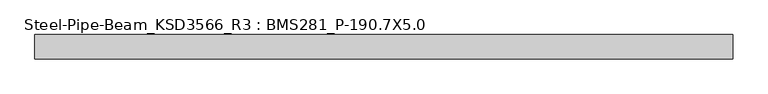
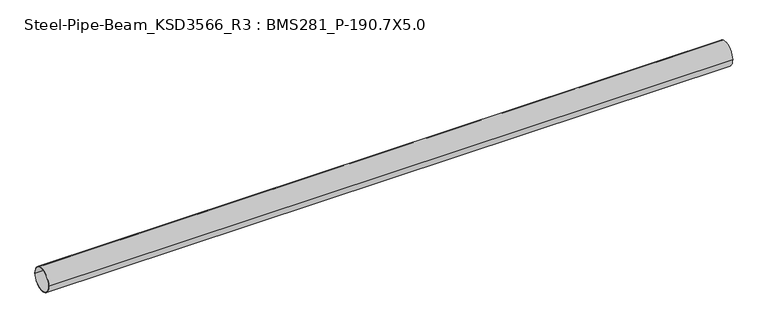
"""IFC4 building model written with IfcOpenShell, lengths in millimetres: member geometry, Steel-Pipe-Beam_KSD3566_R3 : BMS281_P-190.7X5.0."""

from ifc_helpers import new_model, si_unit, point, frame, origin, origin_2d, place, context, project, spatial, circle_curve, trimmed, segment, composite_curve, outline, extrude, source, transform, mapped, element, save


def steel_pipe_beam_ksd3566_r3_bms281_p_190_7x5_0_8f12f416(model_context):
    return source(origin(), model_context, "Body", "SweptSolid", [
        extrude(outline(composite_curve([segment(trimmed(circle_curve(origin_2d(), 95.35), [point((-95.35, 0.0))], [point((95.35, 0.0))], False, "CARTESIAN"), True, "CONTINUOUS"), segment(trimmed(circle_curve(origin_2d(), 95.35), [point((95.35, 0.0))], [point((-95.35, 0.0))], False, "CARTESIAN"), True, "CONTINUOUS")], self_intersect=False), holes=[composite_curve([segment(trimmed(circle_curve(origin_2d(), 90.35), [point((90.35, 0.0))], [point((-90.35, 0.0))], True, "CARTESIAN"), True, "CONTINUOUS"), segment(trimmed(circle_curve(origin_2d(), 90.35), [point((-90.35, 0.0))], [point((90.35, 0.0))], True, "CARTESIAN"), True, "CONTINUOUS")], self_intersect=False)]), frame((-2743.0186842, 0.0, 0.0), z_axis=(1.0, 0.0, 0.0), x_axis=(0.0, 1.0, 0.0)), (0.0, 0.0, 1.0), 5479.06158),
    ])


if __name__ == "__main__":
    model = new_model("IFC4")
    model_context = context("Model", 3, world=origin())
    ifc_project = project(units=[si_unit("LENGTHUNIT", "METRE", prefix="MILLI")], contexts=[model_context])
    site = spatial("IfcSite", under=ifc_project)
    building = spatial("IfcBuilding", under=site)
    placement = place(None, origin())
    steel_pipe_beam_ksd3566_r3_bms281_p_190_7x5_0_shape = steel_pipe_beam_ksd3566_r3_bms281_p_190_7x5_0_8f12f416(model_context)
    element("IfcMember", 1, ObjectType="Steel-Pipe-Beam_KSD3566_R3 : BMS281_P-190.7X5.0", at=placement, inside=building, context=model_context, shape_type="MappedRepresentation", body=[
        mapped(steel_pipe_beam_ksd3566_r3_bms281_p_190_7x5_0_shape, transform((0.0, 0.0, 0.0), x_axis=(1.0, 0.0, 0.0), y_axis=(0.0, 1.0, 0.0), z_axis=(0.0, 0.0, 1.0))),
    ])
    save(model, "model.ifc")

# Revit data of these elements
# Type "Steel-Pipe-Beam_KSD3566_R3 : BMS281_P-190.7X5.0"
#   Keynote = "P-190.7X5.0"
#   SteelWeight = "Light"
#   t = 0.0050 m
#   Surface Area = 0.599102 m²/m
#   Section Area = 29.1697 cm²
#   Mass per Unit Length = 22.8982 kg/m
#   Length [instance default] = 1.5000 m
#   D = 0.1907 m
#   hec_material4 [instance default] = none
#   hec_material3 [instance default] = none
#   hec_material2 [instance default] = none
#   hec_material1 [instance default] = none
#   Structural Material [instance default] = Steel, 45-345
#   Assembly Code = ""
# Element 1 (IfcMember, "Steel-Pipe-Beam_KSD3566_R3 : BMS281_P-190.7X5.0")
#   Structural Material = none
# Materials
#   "Steel, 45-345": class "Metal", colour RGB 189 187 185, transparency 0, Description = "Steel 345 MPa", Cost = 0
